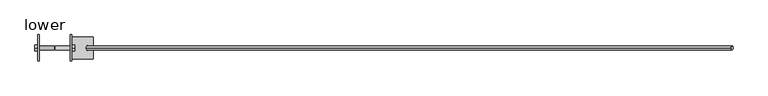
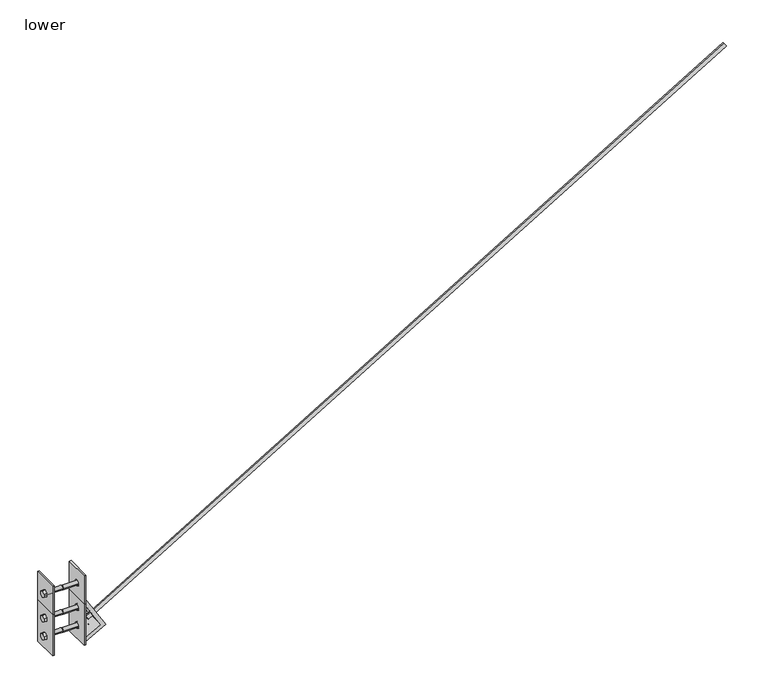
"""IFC4 building model written with IfcOpenShell, lengths in millimetres: fastener geometry, 060523 - W_P_C - Fastenings - Column Base & Top with X Bracing - Custom : lower."""

from ifc_helpers import new_model, si_unit, point, frame, frame_2d, origin, place, context, project, spatial, polyline, circle_curve, trimmed, segment, composite_curve, outline, extrude, source, transform, mapped, element, save
from ifc_brep_helpers import plane_surface, revolved_surface, advanced_brep


def lower_6a7a9d34(model_context):
    return source(origin(), model_context, "Body", "SolidModel", [
        extrude(outline(polyline([(14.2875, 168.586392), (14.2875, 152.088608), (0.0, 143.8397161), (-14.2875, 152.088608), (-14.2875, 168.586392), (0.0, 176.8352839), (14.2875, 168.586392)])), frame((-90.4875, 0.0, 0.0), z_axis=(1.0, 0.0, 0.0), x_axis=(0.0, 1.0, 0.0)), (0.0, 0.0, 1.0), 12.7),
        extrude(outline(composite_curve([segment(trimmed(circle_curve(frame_2d((0.0, 160.3375)), 9.525), [point((9.525, 160.3375))], [point((-9.525, 160.3375))], False, "CARTESIAN"), True, "CONTINUOUS"), segment(trimmed(circle_curve(frame_2d((0.0, 160.3375)), 9.525), [point((-9.525, 160.3375))], [point((9.525, 160.3375))], False, "CARTESIAN"), True, "CONTINUOUS")], self_intersect=False)), frame((-77.7875, 0.0, 0.0), z_axis=(1.0, 0.0, 0.0), x_axis=(0.0, 1.0, 0.0)), (0.0, 0.0, 1.0), 76.2),
        extrude(outline(polyline([(14.2875, 79.686392), (14.2875, 63.188608), (0.0, 54.9397161), (-14.2875, 63.188608), (-14.2875, 79.686392), (0.0, 87.9352839), (14.2875, 79.686392)])), frame((-90.4875, 0.0, 0.0), z_axis=(1.0, 0.0, 0.0), x_axis=(0.0, 1.0, 0.0)), (0.0, 0.0, 1.0), 12.7),
        extrude(outline(composite_curve([segment(trimmed(circle_curve(frame_2d((0.0, 71.4375)), 9.525), [point((9.525, 71.4375))], [point((-9.525, 71.4375))], False, "CARTESIAN"), True, "CONTINUOUS"), segment(trimmed(circle_curve(frame_2d((0.0, 71.4375)), 9.525), [point((-9.525, 71.4375))], [point((9.525, 71.4375))], False, "CARTESIAN"), True, "CONTINUOUS")], self_intersect=False)), frame((-77.7875, 0.0, 0.0), z_axis=(1.0, 0.0, 0.0), x_axis=(0.0, 1.0, 0.0)), (0.0, 0.0, 1.0), 76.2),
        extrude(outline(polyline([(14.2875, 168.586392), (14.2875, 152.088608), (0.0, 143.8397161), (-14.2875, 152.088608), (-14.2875, 168.586392), (0.0, 176.8352839), (14.2875, 168.586392)])), frame((-90.4875, 0.0, 0.0), z_axis=(1.0, 0.0, 0.0), x_axis=(0.0, 1.0, 0.0)), (0.0, 0.0, 1.0), 12.7),
        extrude(outline(composite_curve([segment(trimmed(circle_curve(frame_2d((0.0, 160.3375)), 9.525), [point((9.525, 160.3375))], [point((-9.525, 160.3375))], False, "CARTESIAN"), True, "CONTINUOUS"), segment(trimmed(circle_curve(frame_2d((0.0, 160.3375)), 9.525), [point((-9.525, 160.3375))], [point((9.525, 160.3375))], False, "CARTESIAN"), True, "CONTINUOUS")], self_intersect=False)), frame((-77.7875, 0.0, 0.0), z_axis=(1.0, 0.0, 0.0), x_axis=(0.0, 1.0, 0.0)), (0.0, 0.0, 1.0), 76.2),
        advanced_brep(
        [(-77.7875, -60.325, 211.1375), (-77.7875, -52.3875, 211.1375), (-77.7875, 60.325, 211.1375), (-77.7875, 60.325, 7.9375), (-77.7875, -52.3875, 7.9375), (-77.7875, -60.325, 7.9375), (-77.7875, -13.890625, 160.3375), (-77.7875, 13.890625, 160.3375), (-77.7875, -13.890625, 71.4375), (-77.7875, 13.890625, 71.4375), (-69.85, 13.890625, 160.3375), (-69.85, -13.890625, 160.3375), (-69.85, 13.890625, 71.4375), (-69.85, -13.890625, 71.4375), (-69.85, -60.325, 211.1375), (-69.85, -60.325, 7.9375), (-69.85, 60.325, 7.9375), (-69.85, 60.325, 211.1375)],
        [
            (0, 1),
            (1, 2),
            (2, 3),
            (3, 4),
            (4, 5),
            (5, 0),
            (6, 7, circle_curve(frame((-77.7875, 0.0, 160.3375), z_axis=(1.0, 0.0, 0.0), x_axis=(0.0, -1.0, 0.0)), 13.890625)),
            (7, 6, circle_curve(frame((-77.7875, 0.0, 160.3375), z_axis=(1.0, 0.0, 0.0), x_axis=(0.0, -1.0, 0.0)), 13.890625)),
            (8, 9, circle_curve(frame((-77.7875, 0.0, 71.4375), z_axis=(1.0, 0.0, 0.0), x_axis=(0.0, -1.0, 0.0)), 13.890625)),
            (9, 8, circle_curve(frame((-77.7875, 0.0, 71.4375), z_axis=(1.0, 0.0, 0.0), x_axis=(0.0, -1.0, 0.0)), 13.890625)),
            (10, 7),
            (6, 11),
            (11, 10, circle_curve(frame((-69.85, 0.0, 160.3375), z_axis=(1.0, 0.0, 0.0), x_axis=(0.0, -1.0, 0.0)), 13.890625)),
            (10, 11, circle_curve(frame((-69.85, 0.0, 160.3375), z_axis=(1.0, 0.0, 0.0), x_axis=(0.0, -1.0, 0.0)), 13.890625)),
            (9, 12),
            (12, 13, circle_curve(frame((-69.85, 0.0, 71.4375), z_axis=(1.0, 0.0, 0.0), x_axis=(0.0, -1.0, 0.0)), 13.890625)),
            (13, 8),
            (13, 12, circle_curve(frame((-69.85, 0.0, 71.4375), z_axis=(1.0, 0.0, 0.0), x_axis=(0.0, -1.0, 0.0)), 13.890625)),
            (14, 15),
            (15, 16),
            (16, 17),
            (17, 14),
            (0, 14),
            (17, 2),
            (16, 3),
            (15, 5),
        ],
        [
            plane_surface(frame((-77.7875, 60.325, 211.1375), z_axis=(-1.0, 0.0, 0.0), x_axis=(0.0, 1.0, 0.0))),
            revolved_surface(polyline([(-77.7875, -13.890625, 160.3375), (-69.85, -13.890625, 160.3375)]), (-69.85, 0.0, 160.3375), (-1.0, 0.0, 0.0)),
            revolved_surface(polyline([(-77.7875, -13.890625, 71.4375), (-69.85, -13.890625, 71.4375)]), (-69.85, 0.0, 71.4375), (-1.0, 0.0, 0.0)),
            plane_surface(frame((-69.85, 60.325, 211.1375), z_axis=(1.0, 0.0, 0.0), x_axis=(0.0, -1.0, 0.0))),
            plane_surface(frame((-77.7875, -60.325, 211.1375), z_axis=(0.0, 0.0, 1.0), x_axis=(1.0, 0.0, 0.0))),
            plane_surface(frame((-77.7875, 60.325, 211.1375), z_axis=(0.0, 1.0, 0.0), x_axis=(1.0, 0.0, 0.0))),
            plane_surface(frame((-77.7875, 60.325, 7.9375), z_axis=(0.0, 0.0, -1.0), x_axis=(1.0, 0.0, 0.0))),
            plane_surface(frame((-77.7875, -60.325, 7.9375), z_axis=(0.0, -1.0, 0.0), x_axis=(1.0, 0.0, 0.0))),
        ],
        [
            (0, [[1, 2, 3, 4, 5, 6], [7, 8], [9, 10]]),
            (1, [[11, -7, 12, 13]]),
            (1, [[-11, 14, -12, -8]]),
            (2, [[15, 16, 17, -10]]),
            (2, [[-15, -9, -17, 18]]),
            (3, [[19, 20, 21, 22], [-13, -14], [-18, -16]]),
            (4, [[-2, -1, 23, -22, 24]]),
            (5, [[-3, -24, -21, 25]]),
            (6, [[-5, -4, -25, -20, 26]]),
            (7, [[-6, -26, -19, -23]]),
        ],
    ),
        extrude(outline(polyline([(14.2875, 168.586392), (14.2875, 152.088608), (0.0, 143.8397161), (-14.2875, 152.088608), (-14.2875, 168.586392), (0.0, 176.8352839), (14.2875, 168.586392)])), frame((77.7875, 0.0, 0.0), z_axis=(1.0, 0.0, 0.0), x_axis=(0.0, 1.0, 0.0)), (0.0, 0.0, 1.0), 12.7),
        extrude(outline(composite_curve([segment(trimmed(circle_curve(frame_2d((0.0, 160.3375)), 9.525), [point((9.525, 160.3375))], [point((-9.525, 160.3375))], False, "CARTESIAN"), True, "CONTINUOUS"), segment(trimmed(circle_curve(frame_2d((0.0, 160.3375)), 9.525), [point((-9.525, 160.3375))], [point((9.525, 160.3375))], False, "CARTESIAN"), True, "CONTINUOUS")], self_intersect=False)), frame((1.5875, 0.0, 0.0), z_axis=(1.0, 0.0, 0.0), x_axis=(0.0, 1.0, 0.0)), (0.0, 0.0, 1.0), 76.2),
        extrude(outline(polyline([(14.2875, 79.686392), (14.2875, 63.188608), (0.0, 54.9397161), (-14.2875, 63.188608), (-14.2875, 79.686392), (0.0, 87.9352839), (14.2875, 79.686392)])), frame((77.7875, 0.0, 0.0), z_axis=(1.0, 0.0, 0.0), x_axis=(0.0, 1.0, 0.0)), (0.0, 0.0, 1.0), 12.7),
        extrude(outline(composite_curve([segment(trimmed(circle_curve(frame_2d((0.0, 71.4375)), 9.525), [point((9.525, 71.4375))], [point((-9.525, 71.4375))], False, "CARTESIAN"), True, "CONTINUOUS"), segment(trimmed(circle_curve(frame_2d((0.0, 71.4375)), 9.525), [point((-9.525, 71.4375))], [point((9.525, 71.4375))], False, "CARTESIAN"), True, "CONTINUOUS")], self_intersect=False)), frame((1.5875, 0.0, 0.0), z_axis=(1.0, 0.0, 0.0), x_axis=(0.0, 1.0, 0.0)), (0.0, 0.0, 1.0), 76.2),
        extrude(outline(polyline([(14.2875, 168.586392), (14.2875, 152.088608), (0.0, 143.8397161), (-14.2875, 152.088608), (-14.2875, 168.586392), (0.0, 176.8352839), (14.2875, 168.586392)])), frame((77.7875, 0.0, 0.0), z_axis=(1.0, 0.0, 0.0), x_axis=(0.0, 1.0, 0.0)), (0.0, 0.0, 1.0), 12.7),
        extrude(outline(composite_curve([segment(trimmed(circle_curve(frame_2d((0.0, 160.3375)), 9.525), [point((9.525, 160.3375))], [point((-9.525, 160.3375))], False, "CARTESIAN"), True, "CONTINUOUS"), segment(trimmed(circle_curve(frame_2d((0.0, 160.3375)), 9.525), [point((-9.525, 160.3375))], [point((9.525, 160.3375))], False, "CARTESIAN"), True, "CONTINUOUS")], self_intersect=False)), frame((1.5875, 0.0, 0.0), z_axis=(1.0, 0.0, 0.0), x_axis=(0.0, 1.0, 0.0)), (0.0, 0.0, 1.0), 76.2),
        advanced_brep(
        [(77.7875, -60.325, 211.1375), (77.7875, -60.325, 7.9375), (77.7875, -52.3875, 7.9375), (77.7875, 60.325, 7.9375), (77.7875, 60.325, 211.1375), (77.7875, -52.3875, 211.1375), (77.7875, -13.890625, 71.4375), (77.7875, 13.890625, 71.4375), (77.7875, -13.890625, 160.3375), (77.7875, 13.890625, 160.3375), (69.85, 13.890625, 160.3375), (69.85, -13.890625, 160.3375), (69.85, -13.890625, 71.4375), (69.85, 13.890625, 71.4375), (69.85, -60.325, 211.1375), (69.85, 60.325, 211.1375), (69.85, 60.325, 7.9375), (69.85, -60.325, 7.9375)],
        [
            (0, 1),
            (1, 2),
            (2, 3),
            (3, 4),
            (4, 5),
            (5, 0),
            (6, 7, circle_curve(frame((77.7875, 0.0, 71.4375), z_axis=(-1.0, 0.0, 0.0), x_axis=(0.0, -1.0, 0.0)), 13.890625)),
            (7, 6, circle_curve(frame((77.7875, 0.0, 71.4375), z_axis=(-1.0, 0.0, 0.0), x_axis=(0.0, -1.0, 0.0)), 13.890625)),
            (8, 9, circle_curve(frame((77.7875, 0.0, 160.3375), z_axis=(-1.0, 0.0, 0.0), x_axis=(0.0, -1.0, 0.0)), 13.890625)),
            (9, 8, circle_curve(frame((77.7875, 0.0, 160.3375), z_axis=(-1.0, 0.0, 0.0), x_axis=(0.0, -1.0, 0.0)), 13.890625)),
            (10, 11, circle_curve(frame((69.85, 0.0, 160.3375), z_axis=(-1.0, 0.0, 0.0), x_axis=(0.0, -1.0, 0.0)), 13.890625)),
            (11, 8),
            (9, 10),
            (11, 10, circle_curve(frame((69.85, 0.0, 160.3375), z_axis=(-1.0, 0.0, 0.0), x_axis=(0.0, -1.0, 0.0)), 13.890625)),
            (6, 12),
            (12, 13, circle_curve(frame((69.85, 0.0, 71.4375), z_axis=(-1.0, 0.0, 0.0), x_axis=(0.0, -1.0, 0.0)), 13.890625)),
            (13, 7),
            (13, 12, circle_curve(frame((69.85, 0.0, 71.4375), z_axis=(-1.0, 0.0, 0.0), x_axis=(0.0, -1.0, 0.0)), 13.890625)),
            (14, 15),
            (15, 16),
            (16, 17),
            (17, 14),
            (4, 15),
            (14, 0),
            (3, 16),
            (1, 17),
        ],
        [
            plane_surface(frame((77.7875, 60.325, 211.1375), z_axis=(1.0, 0.0, 0.0), x_axis=(0.0, 1.0, 0.0))),
            revolved_surface(polyline([(77.7875, -13.890625, 160.3375), (69.85, -13.890625, 160.3375)]), (69.85, 0.0, 160.3375), (1.0, 0.0, 0.0)),
            revolved_surface(polyline([(77.7875, -13.890625, 71.4375), (69.85, -13.890625, 71.4375)]), (69.85, 0.0, 71.4375), (1.0, 0.0, 0.0)),
            plane_surface(frame((69.85, 60.325, 211.1375), z_axis=(-1.0, 0.0, 0.0), x_axis=(0.0, -1.0, 0.0))),
            plane_surface(frame((77.7875, -60.325, 211.1375), z_axis=(0.0, 0.0, 1.0), x_axis=(-1.0, 0.0, 0.0))),
            plane_surface(frame((77.7875, 60.325, 211.1375), z_axis=(0.0, 1.0, 0.0), x_axis=(-1.0, 0.0, 0.0))),
            plane_surface(frame((77.7875, 60.325, 7.9375), z_axis=(0.0, 0.0, -1.0), x_axis=(-1.0, 0.0, 0.0))),
            plane_surface(frame((77.7875, -60.325, 7.9375), z_axis=(0.0, -1.0, 0.0), x_axis=(-1.0, 0.0, 0.0))),
        ],
        [
            (0, [[1, 2, 3, 4, 5, 6], [7, 8], [9, 10]]),
            (1, [[11, 12, -10, 13]]),
            (1, [[-9, -12, 14, -13]]),
            (2, [[-7, 15, 16, 17]]),
            (2, [[18, -15, -8, -17]]),
            (3, [[19, 20, 21, 22], [-16, -18], [-14, -11]]),
            (4, [[23, -19, 24, -6, -5]]),
            (5, [[25, -20, -23, -4]]),
            (6, [[26, -21, -25, -3, -2]]),
            (7, [[-24, -22, -26, -1]]),
        ],
    ),
        extrude(outline(polyline([(14.2875, 289.236392), (14.2875, 272.738608), (0.0, 264.4897161), (-14.2875, 272.738608), (-14.2875, 289.236392), (0.0, 297.4852839), (14.2875, 289.236392)])), frame((-90.4875, 0.0, 0.0), z_axis=(1.0, 0.0, 0.0), x_axis=(0.0, 1.0, 0.0)), (0.0, 0.0, 1.0), 12.7),
        extrude(outline(composite_curve([segment(trimmed(circle_curve(frame_2d((0.0, 280.9875)), 9.525), [point((9.525, 280.9875))], [point((-9.525, 280.9875))], False, "CARTESIAN"), True, "CONTINUOUS"), segment(trimmed(circle_curve(frame_2d((0.0, 280.9875)), 9.525), [point((-9.525, 280.9875))], [point((9.525, 280.9875))], False, "CARTESIAN"), True, "CONTINUOUS")], self_intersect=False)), frame((-77.7875, 0.0, 0.0), z_axis=(1.0, 0.0, 0.0), x_axis=(0.0, 1.0, 0.0)), (0.0, 0.0, 1.0), 76.2),
        advanced_brep(
        [(-77.7875, -60.325, 350.8375), (-77.7875, 52.3875, 350.8375), (-77.7875, 60.325, 350.8375), (-77.7875, 60.325, 211.1375), (-77.7875, 52.3875, 211.1375), (-77.7875, -60.325, 211.1375), (-77.7875, -13.890625, 280.9875), (-77.7875, 13.890625, 280.9875), (-69.85, -60.325, 350.8375), (-69.85, -60.325, 211.1375), (-69.85, 60.325, 211.1375), (-69.85, 60.325, 350.8375), (-69.85, 13.890625, 280.9875), (-69.85, -13.890625, 280.9875)],
        [
            (0, 1),
            (1, 2),
            (2, 3),
            (3, 4),
            (4, 5),
            (5, 0),
            (6, 7, circle_curve(frame((-77.7875, 0.0, 280.9875), z_axis=(1.0, 0.0, 0.0), x_axis=(0.0, -1.0, 0.0)), 13.890625)),
            (7, 6, circle_curve(frame((-77.7875, 0.0, 280.9875), z_axis=(1.0, 0.0, 0.0), x_axis=(0.0, -1.0, 0.0)), 13.890625)),
            (8, 9),
            (9, 10),
            (10, 11),
            (11, 8),
            (12, 13, circle_curve(frame((-69.85, 0.0, 280.9875), z_axis=(-1.0, 0.0, 0.0), x_axis=(0.0, -1.0, 0.0)), 13.890625)),
            (13, 12, circle_curve(frame((-69.85, 0.0, 280.9875), z_axis=(-1.0, 0.0, 0.0), x_axis=(0.0, -1.0, 0.0)), 13.890625)),
            (0, 8),
            (11, 2),
            (10, 3),
            (9, 5),
            (12, 7),
            (6, 13),
        ],
        [
            plane_surface(frame((-77.7875, 60.325, 350.8375), z_axis=(-1.0, 0.0, 0.0), x_axis=(0.0, 1.0, 0.0))),
            plane_surface(frame((-69.85, 60.325, 350.8375), z_axis=(1.0, 0.0, 0.0), x_axis=(0.0, -1.0, 0.0))),
            plane_surface(frame((-77.7875, -60.325, 350.8375), z_axis=(0.0, 0.0, 1.0), x_axis=(1.0, 0.0, 0.0))),
            plane_surface(frame((-77.7875, 60.325, 350.8375), z_axis=(0.0, 1.0, 0.0), x_axis=(1.0, 0.0, 0.0))),
            plane_surface(frame((-77.7875, 60.325, 211.1375), z_axis=(0.0, 0.0, -1.0), x_axis=(1.0, 0.0, 0.0))),
            plane_surface(frame((-77.7875, -60.325, 211.1375), z_axis=(0.0, -1.0, 0.0), x_axis=(1.0, 0.0, 0.0))),
            revolved_surface(polyline([(-77.7875, -13.890625, 280.9875), (-69.85, -13.890625, 280.9875)]), (-69.85, 0.0, 280.9875), (-1.0, 0.0, 0.0)),
        ],
        [
            (0, [[1, 2, 3, 4, 5, 6], [7, 8]]),
            (1, [[9, 10, 11, 12], [13, 14]]),
            (2, [[-2, -1, 15, -12, 16]]),
            (3, [[-3, -16, -11, 17]]),
            (4, [[-5, -4, -17, -10, 18]]),
            (5, [[-6, -18, -9, -15]]),
            (6, [[19, -7, 20, -13]]),
            (6, [[-19, -14, -20, -8]]),
        ],
    ),
        extrude(outline(polyline([(14.2875, 289.236392), (14.2875, 272.738608), (0.0, 264.4897161), (-14.2875, 272.738608), (-14.2875, 289.236392), (0.0, 297.4852839), (14.2875, 289.236392)])), frame((77.7875, 0.0, 0.0), z_axis=(1.0, 0.0, 0.0), x_axis=(0.0, 1.0, 0.0)), (0.0, 0.0, 1.0), 12.7),
        extrude(outline(composite_curve([segment(trimmed(circle_curve(frame_2d((0.0, 280.9875)), 9.525), [point((9.525, 280.9875))], [point((-9.525, 280.9875))], False, "CARTESIAN"), True, "CONTINUOUS"), segment(trimmed(circle_curve(frame_2d((0.0, 280.9875)), 9.525), [point((-9.525, 280.9875))], [point((9.525, 280.9875))], False, "CARTESIAN"), True, "CONTINUOUS")], self_intersect=False)), frame((1.5875, 0.0, 0.0), z_axis=(1.0, 0.0, 0.0), x_axis=(0.0, 1.0, 0.0)), (0.0, 0.0, 1.0), 76.2),
        advanced_brep(
        [(77.7875, -60.325, 350.8375), (77.7875, -60.325, 211.1375), (77.7875, 52.3875, 211.1375), (77.7875, 60.325, 211.1375), (77.7875, 60.325, 350.8375), (77.7875, 52.3875, 350.8375), (77.7875, -13.890625, 280.9875), (77.7875, 13.890625, 280.9875), (69.85, -60.325, 350.8375), (69.85, 60.325, 350.8375), (69.85, 60.325, 211.1375), (69.85, -60.325, 211.1375), (69.85, 13.890625, 280.9875), (69.85, -13.890625, 280.9875)],
        [
            (0, 1),
            (1, 2),
            (2, 3),
            (3, 4),
            (4, 5),
            (5, 0),
            (6, 7, circle_curve(frame((77.7875, 0.0, 280.9875), z_axis=(-1.0, 0.0, 0.0), x_axis=(0.0, -1.0, 0.0)), 13.890625)),
            (7, 6, circle_curve(frame((77.7875, 0.0, 280.9875), z_axis=(-1.0, 0.0, 0.0), x_axis=(0.0, -1.0, 0.0)), 13.890625)),
            (8, 9),
            (9, 10),
            (10, 11),
            (11, 8),
            (12, 13, circle_curve(frame((69.85, 0.0, 280.9875), z_axis=(1.0, 0.0, 0.0), x_axis=(0.0, -1.0, 0.0)), 13.890625)),
            (13, 12, circle_curve(frame((69.85, 0.0, 280.9875), z_axis=(1.0, 0.0, 0.0), x_axis=(0.0, -1.0, 0.0)), 13.890625)),
            (4, 9),
            (8, 0),
            (3, 10),
            (1, 11),
            (13, 6),
            (7, 12),
        ],
        [
            plane_surface(frame((77.7875, 60.325, 350.8375), z_axis=(1.0, 0.0, 0.0), x_axis=(0.0, 1.0, 0.0))),
            plane_surface(frame((69.85, 60.325, 350.8375), z_axis=(-1.0, 0.0, 0.0), x_axis=(0.0, -1.0, 0.0))),
            plane_surface(frame((77.7875, -60.325, 350.8375), z_axis=(0.0, 0.0, 1.0), x_axis=(-1.0, 0.0, 0.0))),
            plane_surface(frame((77.7875, 60.325, 350.8375), z_axis=(0.0, 1.0, 0.0), x_axis=(-1.0, 0.0, 0.0))),
            plane_surface(frame((77.7875, 60.325, 211.1375), z_axis=(0.0, 0.0, -1.0), x_axis=(-1.0, 0.0, 0.0))),
            plane_surface(frame((77.7875, -60.325, 211.1375), z_axis=(0.0, -1.0, 0.0), x_axis=(-1.0, 0.0, 0.0))),
            revolved_surface(polyline([(77.7875, -13.890625, 280.9875), (69.85, -13.890625, 280.9875)]), (69.85, 0.0, 280.9875), (1.0, 0.0, 0.0)),
        ],
        [
            (0, [[1, 2, 3, 4, 5, 6], [7, 8]]),
            (1, [[9, 10, 11, 12], [13, 14]]),
            (2, [[15, -9, 16, -6, -5]]),
            (3, [[17, -10, -15, -4]]),
            (4, [[18, -11, -17, -3, -2]]),
            (5, [[-16, -12, -18, -1]]),
            (6, [[-14, 19, -8, 20]]),
            (6, [[-7, -19, -13, -20]]),
        ],
    ),
        extrude(outline(composite_curve([segment(trimmed(circle_curve(frame_2d((0.0, 9.525)), 9.525), [point((0.0, 19.05))], [point((0.0, 0.0))], False, "CARTESIAN"), True, "CONTINUOUS"), segment(trimmed(circle_curve(frame_2d((0.0, 9.525)), 9.525), [point((0.0, 0.0))], [point((0.0, 19.05))], False, "CARTESIAN"), True, "CONTINUOUS")], self_intersect=False)), frame((121.5297809, 0.0, 84.6558969), z_axis=(0.8571673007021132, 0.0, 0.5150380749100526), x_axis=(0.0, 1.0, 0.0)), (0.0, 0.0, 1.0), 3467.1),
        advanced_brep(
        [(175.4460516, 50.8, 68.8992672), (77.7875, 50.8, 15.875), (77.7875, 50.8, 33.9390543), (153.29752, 50.8, 74.93765), (77.7875, 50.8, 200.6074271), (77.7875, 50.8, 231.430391), (175.4460516, -50.8, 68.8992672), (77.7875, -50.8, 231.430391), (77.7875, -50.8, 200.6074271), (153.29752, -50.8, 74.93765), (77.7875, -50.8, 33.9390543), (77.7875, -50.8, 15.875), (154.8010723, 0.0, 103.2582828), (143.7631626, 0.0, 121.6284495), (130.1556317, 0.0, 113.45222), (141.1935414, 0.0, 95.0820533), (123.5760275, 0.0, 58.8001963), (122.8784665, 0.0, 58.4214515), (130.4533618, 0.0, 44.4702298), (131.1509229, 0.0, 44.8489746)],
        [
            (0, 1),
            (1, 2),
            (2, 3),
            (3, 4),
            (4, 5),
            (5, 0),
            (6, 7),
            (7, 8),
            (8, 9),
            (9, 10),
            (10, 11),
            (11, 6),
            (5, 7),
            (6, 0),
            (12, 13, circle_curve(frame((149.2821174, 0.0, 112.4433661), z_axis=(-0.8571673007021132, 0.0, -0.5150380749100526), x_axis=(-0.5150380749100526, 0.0, 0.8571673007021132)), 10.715625)),
            (13, 12, circle_curve(frame((149.2821174, 0.0, 112.4433661), z_axis=(-0.8571673007021132, 0.0, -0.5150380749100526), x_axis=(-0.5150380749100526, 0.0, 0.8571673007021132)), 10.715625)),
            (4, 8),
            (3, 9),
            (14, 15, circle_curve(frame((135.6745865, 0.0, 104.2671367), z_axis=(0.8571673007021132, 0.0, 0.5150380749100526), x_axis=(-0.5150380749100526, 0.0, 0.8571673007021132)), 10.715625)),
            (15, 14, circle_curve(frame((135.6745865, 0.0, 104.2671367), z_axis=(0.8571673007021132, 0.0, 0.5150380749100526), x_axis=(-0.5150380749100526, 0.0, 0.8571673007021132)), 10.715625)),
            (2, 10),
            (16, 17, circle_curve(frame((123.227247, 0.0, 58.6108239), z_axis=(0.47715876025960574, 0.0, -0.8788171126619669), x_axis=(0.8788171126619669, 0.0, 0.47715876025960574)), 0.396875)),
            (17, 16, circle_curve(frame((123.227247, 0.0, 58.6108239), z_axis=(0.47715876025960574, 0.0, -0.8788171126619669), x_axis=(0.8788171126619669, 0.0, 0.47715876025960574)), 0.396875)),
            (1, 11),
            (18, 19, circle_curve(frame((130.8021423, 0.0, 44.6596022), z_axis=(-0.47715876025960574, 0.0, 0.8788171126619669), x_axis=(0.8788171126619669, 0.0, 0.47715876025960574)), 0.396875)),
            (19, 18, circle_curve(frame((130.8021423, 0.0, 44.6596022), z_axis=(-0.47715876025960574, 0.0, 0.8788171126619669), x_axis=(0.8788171126619669, 0.0, 0.47715876025960574)), 0.396875)),
            (13, 14),
            (15, 12),
            (19, 16),
            (17, 18),
        ],
        [
            plane_surface(frame((77.7875, 50.8, 231.430391), z_axis=(0.0, 1.0, 0.0), x_axis=(-0.5150380749100526, 0.0, 0.8571673007021132))),
            plane_surface(frame((77.7875, -50.8, 231.430391), z_axis=(0.0, -1.0, 0.0), x_axis=(0.5150380749100526, 0.0, -0.8571673007021132))),
            plane_surface(frame((175.4460516, 50.8, 68.8992672), z_axis=(0.8571673007021132, 0.0, 0.5150380749100526), x_axis=(0.0, -1.0, 0.0))),
            plane_surface(frame((77.7875, 50.8, 231.430391), z_axis=(-1.0, 0.0, 0.0), x_axis=(0.0, -1.0, 0.0))),
            plane_surface(frame((77.7875, 50.8, 200.6074271), z_axis=(-0.8571673007021139, 0.0, -0.5150380749100517), x_axis=(0.0, -1.0, 0.0))),
            plane_surface(frame((153.29752, 50.8, 74.93765), z_axis=(-0.47715876025960563, 0.0, 0.8788171126619669), x_axis=(0.0, -1.0, 0.0))),
            plane_surface(frame((77.7875, 50.8, 33.9390543), z_axis=(-1.0, 0.0, 0.0), x_axis=(0.0, -1.0, 0.0))),
            plane_surface(frame((77.7875, 50.8, 15.875), z_axis=(0.477158760259606, 0.0, -0.8788171126619667), x_axis=(0.0, -1.0, 0.0))),
            revolved_surface(polyline([(130.15563164620562, 0.0, 113.45222002718884), (143.76316260021085, 0.0, 121.62844949964908)]), (149.2821174, 0.0, 112.4433661), (-0.8571673007021132, 0.0, -0.5150380749100526)),
            revolved_surface(polyline([(123.57602749491133, 0.0, 58.80019629723708), (131.15092285819438, 0.0, 44.848974552392434)]), (130.8021423, 0.0, 44.6596022), (-0.47715876025960574, 0.0, 0.8788171126619669)),
        ],
        [
            (0, [[1, 2, 3, 4, 5, 6]]),
            (1, [[7, 8, 9, 10, 11, 12]]),
            (2, [[13, -7, 14, -6], [15, 16]]),
            (3, [[17, -8, -13, -5]]),
            (4, [[18, -9, -17, -4], [19, 20]]),
            (5, [[21, -10, -18, -3], [22, 23]]),
            (6, [[24, -11, -21, -2]]),
            (7, [[-14, -12, -24, -1], [25, 26]]),
            (8, [[-16, 27, -20, 28]]),
            (8, [[-19, -27, -15, -28]]),
            (9, [[-26, 29, -23, 30]]),
            (9, [[-22, -29, -25, -30]]),
        ],
    ),
    ])


if __name__ == "__main__":
    model = new_model("IFC4")
    model_context = context("Model", 3, world=origin())
    ifc_project = project(units=[si_unit("LENGTHUNIT", "METRE", prefix="MILLI")], contexts=[model_context])
    site = spatial("IfcSite", under=ifc_project)
    building = spatial("IfcBuilding", under=site)
    placement = place(None, origin())
    lower_shape = lower_6a7a9d34(model_context)
    element("IfcFastener", 1, ObjectType="060523 - W_P_C - Fastenings - Column Base & Top with X Bracing - Custom : lower", at=placement, inside=building, context=model_context, shape_type="MappedRepresentation", body=[
        mapped(lower_shape, transform((0.0, 0.0, 0.0), x_axis=(1.0, 0.0, 0.0), y_axis=(0.0, 1.0, 0.0), z_axis=(0.0, 0.0, 1.0))),
    ])
    save(model, "model.ifc")

# Revit data of these elements
# Type "060523 - W_P_C - Fastenings - Column Base & Top with X Bracing - Custom : lower"
#   Width - Top = 0' - 5 1/2"
#   Top/Bottom Plate Thickness = 0' - 0 5/16"
#   Top/Bottom Plate - Width = 0' - 7 1/2"
#   Rod Radius = 0' - 0 3/8"
#   Rod Length [instance default] = 11' - 4"
#   Plate Thickness = 0' - 0 5/16"
#   Offset - Upper Plate 2 = 0' - 0"
#   Height of Plate = 0' - 8"
#   Width - Bottom = 0' - 5 1/2"
#   Plate Width = 0' - 4 3/4"
#   Bracket Width = 0' - 4"
#   Bracket Thickness = 0' - 0 5/8"
#   Bracket Offset in X = 0' - 3 1/16"
#   Bracket Offset in Y = 0' - 0 3/8"
#   Bracket Offset = 0' - 0 5/8"
#   Bracket Leg = 0' - 4 3/8"
#   Bracket Hole Radius - Up = 0' - 0 27/64"
#   Bracket Hole Radius - Down = 0' - 0 1/64"
#   Bracket Hole Offset = 0' - 2"
#   Beam Width = 0' - 7 3/8"
#   Angle 2 = 31.00°
#   Angle 1 = 118.50°
#   Top Plate Visible = no
#   Rod Visibility = yes
#   Plate Visibility - Upper Right 2 = no
#   Plate Visibility - Upper Right 1 = yes
#   Plate Visibility - Upper Left 2 = no
#   Plate Visibility - Upper Left 1 = yes
#   Plate Visibility - Lower Right 2 = no
#   Plate Visibility - Lower Right 1 = yes
#   Plate Visibility - Lower Left 2 = no
#   Plate Visibility - Lower Left 1 = yes
#   Bracket Visibility = yes
#   Bottom Plate Visible = no
#   Upper Plates - 2 = element 1925091
#   Upper Plates - 1 = element 1925091
#   Rod Material = X-BRACING: 3/4" DIA. THREADED STEEL ROD (RAW) W/ TURNBUCKLE (NUTS AT STEEL ANGLE)
#   Lower Plates = element 1925092
#   Bracket Material = 5/8" STEEL ANGLE (RAW STEEL)
#   URL = ""
# Element 1 (IfcFastener, "060523 - W_P_C - Fastenings - Column Base & Top with X Bracing - Custom : lower")
#   Rod Length = 11' - 3"
#   Materials on its faces: "3/4\" LAG BOLT (THRU BOLT IF PLATE ON OPP. SIDE OF STRUCT MEMBER)", "5/16\" STEEL PLATE (RAW STEEL)", "5/8\" STEEL ANGLE (RAW STEEL)", "X-BRACING: 3/4\" DIA. THREADED STEEL ROD (RAW) W/ TURNBUCKLE (NUTS AT STEEL ANGLE)"
# Materials
#   "X-BRACING: 3/4\" DIA. THREADED STEEL ROD (RAW) W/ TURNBUCKLE (NUTS AT STEEL ANGLE)": class "Generic", colour RGB 212 212 212, transparency 0, Cost = 0
#   "5/8\" STEEL ANGLE (RAW STEEL)": class "Generic", colour RGB 195 195 195, transparency 0, Cost = 0
#   "3/4\" LAG BOLT (THRU BOLT IF PLATE ON OPP. SIDE OF STRUCT MEMBER)": class "Generic", colour RGB 120 120 120, transparency 0, Cost = 0
#   "5/16\" STEEL PLATE (RAW STEEL)": class "Generic", colour RGB 232 232 232, transparency 0, Cost = 0
